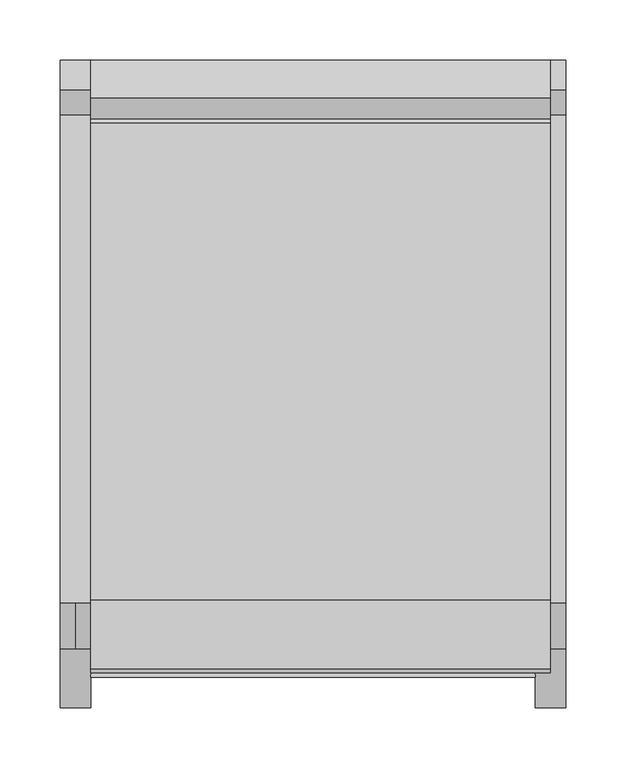
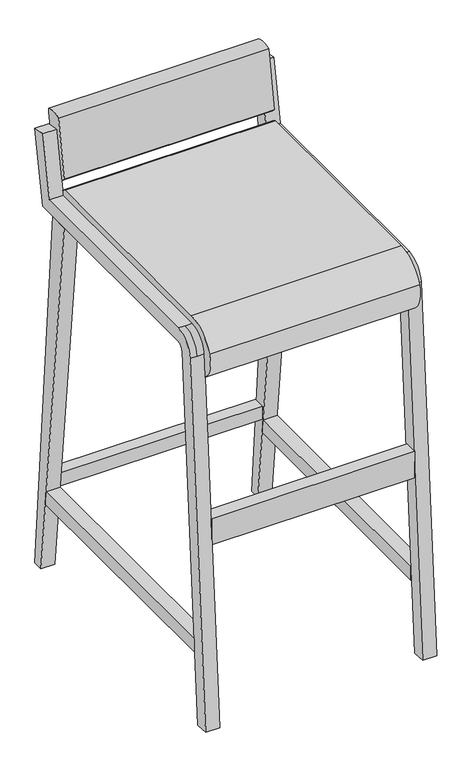
"""IFC4 building model written with IfcOpenShell, lengths in millimetres: furniture geometry, Bar_Stool_6722[1] : Bar_Stool_6722[1]."""

import ifcopenshell
import ifcopenshell.guid

model = None  # the IFC model being written
_history = None  # IfcOwnerHistory: only IFC2X3 demands one
_inside = {}  # id of a spatial element -> (the spatial element, [elements in it])
_under = {}  # id of a project, library or spatial element -> (it, [spatial elements below it])
_declared = {}  # id of a project -> (the project, [libraries it declares])
_typed = {}  # id of a type object -> (the type object, [elements of that type])
_made_of = {}  # id of a material, layer set ... -> (it, [elements and type objects made of it])


def new_model(schema):
    """Start an empty IFC model of exactly this schema.

    Asked for "IFC4X3", IfcOpenShell would pick the latest addendum, in which some entities
    have other attributes; the version numbers below select the first issue.
    IFC2X3 requires an IfcOwnerHistory on every rooted entity: one is made here for all.
    """
    global model, _history
    if schema == "IFC4X3":
        model = ifcopenshell.file(schema_version=(4, 3, 0, 0))
    else:
        model = ifcopenshell.file(schema=schema)
    _inside.clear()
    _under.clear()
    _declared.clear()
    _typed.clear()
    _made_of.clear()
    _history = None
    if model.schema == "IFC2X3":
        org = make("IfcOrganization", Name="unknown")
        user = make(
            "IfcPersonAndOrganization",
            ThePerson=make("IfcPerson", FamilyName="unknown"),
            TheOrganization=org,
        )
        app = make(
            "IfcApplication",
            ApplicationDeveloper=org,
            Version="unknown",
            ApplicationFullName="unknown",
            ApplicationIdentifier="unknown",
        )
        _history = make(
            "IfcOwnerHistory",
            OwningUser=user,
            OwningApplication=app,
            ChangeAction="ADDED",
            CreationDate=0,
        )
    return model


def make(cls, **values):
    """One entity of the class cls with the attributes given. An attribute that is None is left unset."""
    return model.create_entity(
        cls, **{name: value for name, value in values.items() if value is not None}
    )


def rooted(cls, **values):
    """An entity with a GlobalId (a new one), such as an element, a storey or a relation."""
    return make(cls, GlobalId=ifcopenshell.guid.new(), OwnerHistory=_history, **values)


def si_unit(unit_type, name, prefix=None):
    """IfcSIUnit, for example si_unit("LENGTHUNIT", "METRE", prefix="MILLI")."""
    return make("IfcSIUnit", UnitType=unit_type, Prefix=prefix, Name=name)


def assignment(units):
    """IfcUnitAssignment: the units of a project."""
    return None if units is None else make("IfcUnitAssignment", Units=units)


def point(xyz):
    """IfcCartesianPoint."""
    return None if xyz is None else make("IfcCartesianPoint", Coordinates=xyz)


def direction(xyz):
    """IfcDirection."""
    return None if xyz is None else make("IfcDirection", DirectionRatios=xyz)


def frame(location, z_axis=None, x_axis=None):
    """IfcAxis2Placement3D, a coordinate frame: its origin and axes. An axis left out is left unset."""
    return make(
        "IfcAxis2Placement3D",
        Location=point(location),
        Axis=direction(z_axis),
        RefDirection=direction(x_axis),
    )


def frame_2d(location, x_axis=None):
    """IfcAxis2Placement2D, a coordinate frame in the plane: its origin and x axis."""
    return make(
        "IfcAxis2Placement2D", Location=point(location), RefDirection=direction(x_axis)
    )


def origin():
    """The frame at (0, 0, 0) with its axes left unset."""
    return frame((0.0, 0.0, 0.0))


def place(relative_to, where):
    """IfcLocalPlacement: puts the frame where relative to a parent placement (None: the world)."""
    return make(
        "IfcLocalPlacement", PlacementRelTo=relative_to, RelativePlacement=where
    )


def context(
    kind, dimensions, precision=None, world=None, true_north=None, identifier=None
):
    """IfcGeometricRepresentationContext, for example the 3D "Model" context."""
    return make(
        "IfcGeometricRepresentationContext",
        ContextIdentifier=identifier,
        ContextType=kind,
        CoordinateSpaceDimension=dimensions,
        Precision=precision,
        WorldCoordinateSystem=world,
        TrueNorth=true_north,
    )


def project(units=None, contexts=None):
    """IfcProject with its units and contexts."""
    return rooted(
        "IfcProject",
        Name="project",
        RepresentationContexts=contexts,
        UnitsInContext=assignment(units),
    )


def spatial(cls, under=None, at=None, **own):
    """A site, building, storey or space (cls), placed at a placement, below another one or the project."""
    s = rooted(cls, ObjectPlacement=at, **own)
    if under is not None:
        _under.setdefault(under.id(), (under, []))[1].append(s)
    return s


def polyline(points):
    """IfcPolyline through the points."""
    return make("IfcPolyline", Points=[point(p) for p in points])


def circle_curve(where, radius):
    """IfcCircle in the frame where."""
    return make("IfcCircle", Position=where, Radius=radius)


def trimmed(basis, trim1, trim2, sense, master):
    """IfcTrimmedCurve: the piece of a basis curve between two trims."""
    return make(
        "IfcTrimmedCurve",
        BasisCurve=basis,
        Trim1=trim1,
        Trim2=trim2,
        SenseAgreement=sense,
        MasterRepresentation=master,
    )


def segment(curve, same_sense, transition):
    """IfcCompositeCurveSegment."""
    return make(
        "IfcCompositeCurveSegment",
        Transition=transition,
        SameSense=same_sense,
        ParentCurve=curve,
    )


def composite_curve(segments, self_intersect=None):
    """IfcCompositeCurve: segments joined end to end."""
    return make("IfcCompositeCurve", Segments=segments, SelfIntersect=self_intersect)


def outline(outer, holes=None, kind="AREA"):
    """IfcArbitraryClosedProfileDef: a profile drawn as a closed curve; with holes, ...WithVoids."""
    if holes is None:
        return make("IfcArbitraryClosedProfileDef", ProfileType=kind, OuterCurve=outer)
    return make(
        "IfcArbitraryProfileDefWithVoids",
        ProfileType=kind,
        OuterCurve=outer,
        InnerCurves=holes,
    )


def extrude(swept, where, along, depth):
    """IfcExtrudedAreaSolid: the profile swept, set in the frame where, extruded along a direction by depth."""
    return make(
        "IfcExtrudedAreaSolid",
        SweptArea=swept,
        Position=where,
        ExtrudedDirection=direction(along),
        Depth=depth,
    )


def shape(context_of_items, identifier, shape_type, items):
    """IfcShapeRepresentation: the items that make up one representation, for example the "Body"."""
    return make(
        "IfcShapeRepresentation",
        ContextOfItems=context_of_items,
        RepresentationIdentifier=identifier,
        RepresentationType=shape_type,
        Items=items,
    )


def source(mapping_origin, context_of_items, identifier, shape_type, items):
    """IfcRepresentationMap: a shape defined once, which mapped items show again and again."""
    return make(
        "IfcRepresentationMap",
        MappingOrigin=mapping_origin,
        MappedRepresentation=shape(context_of_items, identifier, shape_type, items),
    )


def transform(
    local_origin,
    x_axis=None,
    y_axis=None,
    z_axis=None,
    scale=None,
    scale2=None,
    scale3=None,
    uniform=True,
):
    """IfcCartesianTransformationOperator3D, or its non-uniform kind. x_axis, y_axis, z_axis: its Axis1, 2, 3."""
    if uniform:
        return make(
            "IfcCartesianTransformationOperator3D",
            Axis1=direction(x_axis),
            Axis2=direction(y_axis),
            LocalOrigin=point(local_origin),
            Scale=scale,
            Axis3=direction(z_axis),
        )
    return make(
        "IfcCartesianTransformationOperator3DnonUniform",
        Axis1=direction(x_axis),
        Axis2=direction(y_axis),
        LocalOrigin=point(local_origin),
        Scale=scale,
        Axis3=direction(z_axis),
        Scale2=scale2,
        Scale3=scale3,
    )


def mapped(mapping_source, mapping_target):
    """IfcMappedItem: shows the shape of a source again, moved by a transform."""
    return make(
        "IfcMappedItem", MappingSource=mapping_source, MappingTarget=mapping_target
    )


def made_of(thing, what):
    """Note that an element or type object is made of a material, layer set ...; save() writes the relation."""
    if what is not None:
        _made_of.setdefault(what.id(), (what, []))[1].append(thing)
    return thing


def element(
    cls,
    number,
    at=None,
    inside=None,
    cuts=None,
    type_object=None,
    material=None,
    context=None,
    identifier="Body",
    shape_type=None,
    held_by="IfcProductDefinitionShape",
    body=None,
    shapes=None,
    **own,
):
    """One element of the class cls, such as IfcWall. Its Tag is "e" and its number.

    at: its placement. inside: the storey or other place that contains it. cuts: it is an
    opening in that element (IfcRelVoidsElement). A single representation is given by context,
    identifier, shape_type and body (its items); several are given by shapes. held_by: the class
    of the entity that holds the representations. save() writes the other relations.
    """
    e = rooted(cls, Tag="e%d" % number, ObjectPlacement=at, **own)
    if body is not None:
        shapes = [shape(context, identifier, shape_type, body)]
    if shapes is not None:
        e.Representation = make(held_by, Representations=shapes)
    if inside is not None:
        _inside.setdefault(inside.id(), (inside, []))[1].append(e)
    if cuts is not None:
        rooted(
            "IfcRelVoidsElement", RelatingBuildingElement=cuts, RelatedOpeningElement=e
        )
    if type_object is not None:
        _typed.setdefault(type_object.id(), (type_object, []))[1].append(e)
    return made_of(e, material)


def aggregate(whole, parts):
    """IfcRelAggregates: a whole, such as a stair, and the parts it consists of."""
    return rooted("IfcRelAggregates", RelatingObject=whole, RelatedObjects=parts)


def save(model, path):
    """Write the relations noted so far, then the file.

    IfcRelAggregates (storeys below a building ...), IfcRelContainedInSpatialStructure (elements
    in a storey), IfcRelDefinesByType, IfcRelAssociatesMaterial and IfcRelDeclares: one each for
    every whole, place, type object, material and project.
    """
    for whole, parts in _under.values():
        aggregate(whole, parts)
    for where, things in _inside.values():
        rooted(
            "IfcRelContainedInSpatialStructure",
            RelatedElements=things,
            RelatingStructure=where,
        )
    for kind, things in _typed.values():
        rooted("IfcRelDefinesByType", RelatedObjects=things, RelatingType=kind)
    for what, things in _made_of.values():
        rooted("IfcRelAssociatesMaterial", RelatedObjects=things, RelatingMaterial=what)
    for by, libraries in _declared.values():
        rooted("IfcRelDeclares", RelatingContext=by, RelatedDefinitions=libraries)
    model.write(path)


def plane_surface(at):
    """IfcPlane: the flat surface through the origin of the frame at, square to its z axis."""
    return make("IfcPlane", Position=at)


def cylinder_surface(at, radius):
    """IfcCylindricalSurface: all points at the distance radius from the z axis of the frame at."""
    return make("IfcCylindricalSurface", Position=at, Radius=radius)


def revolved_surface(curve, axis_point, axis_direction):
    """IfcSurfaceOfRevolution: the curve turned about the line through axis_point along axis_direction."""
    return make(
        "IfcSurfaceOfRevolution",
        SweptCurve=make("IfcArbitraryOpenProfileDef", ProfileType="CURVE", Curve=curve),
        AxisPosition=make("IfcAxis1Placement", Location=point(axis_point), Axis=direction(axis_direction)),
    )


def advanced_brep(points, edges, surfaces, faces):
    """IfcAdvancedBrep: a solid bounded by faces that lie on surfaces and meet in shared edges.

    An edge is (start, end): straight between two places in points (the first is 0);
    or (start, end, curve); or (start, end, curve, False) where it runs against its curve.
    A face is (place in surfaces, loops), or (place, loops, False) where it looks against
    its surface's normal. A loop lists edges by number (the first is 1), with a minus sign
    where the edge is run from its end to its start. The first loop is the outer one.
    """
    corners = [point(p) for p in points]
    vertices = [make("IfcVertexPoint", VertexGeometry=c) for c in corners]
    made = []
    for start, end, *more in edges:
        made.append(
            make(
                "IfcEdgeCurve",
                EdgeStart=vertices[start],
                EdgeEnd=vertices[end],
                EdgeGeometry=more[0] if more else make("IfcPolyline", Points=[corners[start], corners[end]]),
                SameSense=more[1] if len(more) > 1 else True,
            )
        )
    hull = []
    for where, loops, *sense in faces:
        bounds = []
        for j, loop in enumerate(loops):
            ring = [make("IfcOrientedEdge", EdgeElement=made[abs(k) - 1], Orientation=k > 0) for k in loop]
            bounds.append(
                make(
                    "IfcFaceOuterBound" if j == 0 else "IfcFaceBound",
                    Bound=make("IfcEdgeLoop", EdgeList=ring),
                    Orientation=True,
                )
            )
        hull.append(make("IfcAdvancedFace", Bounds=bounds, FaceSurface=surfaces[where], SameSense=sense[0] if sense else True))
    return make("IfcAdvancedBrep", Outer=make("IfcClosedShell", CfsFaces=hull))


def furniture_9d95edac(model_context):
    return source(origin(), model_context, "Body", "SolidModel", [
        advanced_brep(
        [(419.1, -25.0141169, 838.4759165), (419.1, 0.0, 834.0652528), (393.7, 0.0, 834.0652528), (393.7, -25.0141169, 838.4759165), (393.7, -45.2169423, 723.9), (419.1, -45.2169423, 723.9), (393.7, -23.9038117, 698.5), (393.7, -450.0350637, 698.5), (393.7, -462.7032819, 686.6979128), (393.7, -511.439502, -0.8979128), (393.7, -536.7759384, 0.8979128), (393.7, -488.0397183, 688.4937383), (393.7, -450.0350637, 723.9), (419.1, -23.9038117, 698.5), (419.1, -450.0350637, 723.9), (419.1, -488.0397183, 688.4937383), (419.1, -536.7759384, 0.8979128), (419.1, -511.439502, -0.8979128), (419.1, -462.7032819, 686.6979128), (419.1, -450.0350637, 698.5), (406.4, -450.0350637, 723.9), (406.4, -488.0397183, 688.4937383)],
        [
            (0, 1),
            (1, 2),
            (2, 3),
            (3, 0),
            (3, 4),
            (4, 5),
            (5, 0),
            (2, 6),
            (6, 7),
            (7, 8, circle_curve(frame((393.7, -450.0350637, 685.8), z_axis=(1.0, 0.0, 0.0), x_axis=(0.0, 0.0, 1.0)), 12.7)),
            (8, 9),
            (9, 10),
            (10, 11),
            (11, 12, circle_curve(frame((393.7, -450.0350637, 685.8), z_axis=(-1.0, 0.0, 0.0), x_axis=(0.0, 0.0, 1.0)), 38.1)),
            (12, 4),
            (1, 13),
            (13, 6),
            (5, 14),
            (14, 15, circle_curve(frame((419.1, -450.0350637, 685.8), z_axis=(1.0, 0.0, 0.0), x_axis=(0.0, 0.0, 1.0)), 38.1)),
            (15, 16),
            (16, 17),
            (17, 18),
            (18, 19, circle_curve(frame((419.1, -450.0350637, 685.8), z_axis=(-1.0, 0.0, 0.0), x_axis=(0.0, 0.0, 1.0)), 12.7)),
            (19, 13),
            (12, 20),
            (20, 14),
            (19, 7),
            (21, 15),
            (20, 21, circle_curve(frame((406.4, -450.0350637, 685.8), z_axis=(1.0, 0.0, 0.0), x_axis=(0.0, 0.0, 1.0)), 38.1)),
            (11, 21),
            (18, 8),
            (10, 16),
            (17, 9),
        ],
        [
            plane_surface(frame((406.4, -12.5070585, 836.2705846), z_axis=(0.0, 0.17364817766692853, 0.9848077530122085), x_axis=(1.0, 0.0, 0.0))),
            plane_surface(frame((406.4, -25.0141169, 838.4759165), z_axis=(0.0, -0.9848077530122085, 0.17364817766692814), x_axis=(0.0, -0.17364817766692814, -0.9848077530122085))),
            plane_surface(frame((393.7, -25.0141169, 838.4759165), z_axis=(-1.0, 0.0, 0.0), x_axis=(0.0, -0.17364817766692808, -0.9848077530122085))),
            plane_surface(frame((393.7, 0.0, 834.0652528), z_axis=(0.0, 0.9848077530122085, -0.17364817766692817), x_axis=(0.0, -0.17364817766692817, -0.9848077530122085))),
            plane_surface(frame((419.1, 0.0, 834.0652528), z_axis=(1.0000000000000002, 0.0, 0.0), x_axis=(0.0, -0.1736481776669284, -0.9848077530122085))),
            plane_surface(frame((406.4, -45.2169423, 723.9), z_axis=(0.0, 0.0, 1.0), x_axis=(0.0, -1.0, 0.0))),
            plane_surface(frame((393.7, -23.9038117, 698.5), z_axis=(0.0, 0.0, -1.0), x_axis=(0.0, -1.0, 0.0))),
            cylinder_surface(frame((406.4, -450.0350637, 685.8), z_axis=(-1.0, 0.0, 0.0), x_axis=(0.0, 0.0, 1.0)), 38.1),
            revolved_surface(polyline([(393.7, -450.0350637, 698.5), (419.1, -450.0350637, 698.5)]), (406.4, -450.0350637, 685.8), (-1.0, 0.0, 0.0)),
            plane_surface(frame((406.4, -488.0397183, 688.4937383), z_axis=(0.0, -0.9974974969901172, 0.07070179275273744), x_axis=(0.0, -0.07070179275273744, -0.9974974969901172))),
            plane_surface(frame((393.7, -462.7032819, 686.6979128), z_axis=(0.0, 0.9974974969901172, -0.07070179275273743), x_axis=(0.0, -0.07070179275273743, -0.9974974969901172))),
            plane_surface(frame((406.4, -524.1077202, 0.0), z_axis=(0.0, -0.07070179275273399, -0.9974974969901175), x_axis=(1.0, 0.0, 0.0))),
        ],
        [
            (0, [[1, 2, 3, 4]]),
            (1, [[-4, 5, 6, 7]]),
            (2, [[8, 9, 10, 11, 12, 13, 14, 15, -5, -3]]),
            (3, [[16, 17, -8, -2]]),
            (4, [[-7, 18, 19, 20, 21, 22, 23, 24, -16, -1]]),
            (5, [[-15, 25, 26, -18, -6]]),
            (6, [[-24, 27, -9, -17]]),
            (7, [[28, -19, -26, 29]]),
            (7, [[30, -29, -25, -14]]),
            (8, [[31, -10, -27, -23]]),
            (9, [[32, -20, -28, -30, -13]]),
            (10, [[33, -11, -31, -22]]),
            (11, [[-12, -33, -21, -32]]),
        ],
    ),
        extrude(outline(composite_curve([segment(polyline([(-48.4096386, 756.5644068), (-31.5225381, 863.1853632)]), True, "CONTINUOUS"), segment(trimmed(circle_curve(frame_2d((-15.7612691, 828.3540875)), 38.2313401), [point((-31.5225381, 863.1853632))], [point((0.0, 863.1853632))], False, "CARTESIAN"), True, "CONTINUOUS"), segment(polyline([(0.0, 863.1853632), (0.0, 856.8353632), (-19.1416957, 748.2774126), (-44.0710693, 752.2258375), (-48.4096386, 756.5644068)]), True, "CONTINUOUS")], self_intersect=False)), frame((25.4, 0.0, 0.0), z_axis=(1.0, 0.0, 0.0), x_axis=(0.0, 1.0, 0.0)), (0.0, 0.0, 1.0), 381.0),
        extrude(outline(composite_curve([segment(polyline([(-51.6744261, 737.5144068), (-43.9498561, 733.0546243), (-46.417441, 704.85), (-452.817441, 704.85), (-460.5585493, 681.23302), (-460.5585493, 643.13302), (-484.2663236, 640.1699505)]), True, "CONTINUOUS"), segment(trimmed(circle_curve(frame_2d((-460.5585493, 681.23302)), 47.4155486), [point((-484.2663236, 640.1699505))], [point((-505.1145904, 697.4500928))], False, "CARTESIAN"), True, "CONTINUOUS"), segment(trimmed(circle_curve(frame_2d((-447.8968201, 676.6245275)), 60.8898793), [point((-505.1145904, 697.4500928))], [point((-447.8968201, 737.5144068))], False, "CARTESIAN"), True, "CONTINUOUS"), segment(polyline([(-447.8968201, 737.5144068), (-51.6744261, 737.5144068)]), True, "CONTINUOUS")], self_intersect=False)), frame((25.4, 0.0, 0.0), z_axis=(1.0, 0.0, 0.0), x_axis=(0.0, 1.0, 0.0)), (0.0, 0.0, 1.0), 381.0),
        extrude(outline(polyline([(393.7, -11.6871233), (393.7, -33.1441574), (25.4, -33.1441574), (25.4, -11.6871233), (393.7, -11.6871233)])), frame((0.0, 0.0, 157.9619127), z_axis=(0.0, 0.0, 1.0), x_axis=(1.0, 0.0, 0.0)), (0.0, 0.0, 1.0), 25.4),
        extrude(outline(polyline([(393.7, -488.2695397), (393.7, -511.439502), (25.4, -511.439502), (25.4, -488.2695397), (393.7, -488.2695397)])), frame((0.0, 0.0, 335.7619127), z_axis=(0.0, 0.0, 1.0), x_axis=(1.0, 0.0, 0.0)), (0.0, 0.0, 1.0), 50.8),
        extrude(outline(polyline([(-500.1796497, 157.9619127), (-35.652466, 157.9619127), (-32.9828185, 132.5619127), (-500.1796497, 132.5619127), (-500.1796497, 157.9619127)])), frame((393.7, 0.0, 0.0), z_axis=(1.0, 0.0, 0.0), x_axis=(0.0, 1.0, 0.0)), (0.0, 0.0, 1.0), 25.4),
        extrude(outline(polyline([(-500.1796497, 157.9619127), (-35.652466, 157.9619127), (-32.9828185, 132.5619127), (-500.1796497, 132.5619127), (-500.1796497, 157.9619127)])), frame((0.0, 0.0, 0.0), z_axis=(1.0, 0.0, 0.0), x_axis=(0.0, 1.0, 0.0)), (0.0, 0.0, 1.0), 25.4),
        extrude(outline(polyline([(0.0, 0.0), (-19.05, 0.0), (-92.4653083, 698.5), (-55.3031462, 698.5), (0.0, 0.0)])), frame((393.7, 0.0, 0.0), z_axis=(1.0, 0.0, 0.0), x_axis=(0.0, 1.0, 0.0)), (0.0, 0.0, 1.0), 25.4),
        advanced_brep(
        [(25.4, -25.0141169, 838.4759165), (25.4, 0.0, 834.0652528), (0.0, 0.0, 834.0652528), (0.0, -25.0141169, 838.4759165), (0.0, -45.2169423, 723.9), (25.4, -45.2169423, 723.9), (0.0, -23.9038117, 698.5), (0.0, -450.0350637, 698.5), (0.0, -462.7032819, 686.6979128), (0.0, -511.439502, -0.8979128), (0.0, -536.7759384, 0.8979128), (0.0, -488.0397183, 688.4937383), (0.0, -450.0350637, 723.9), (25.4, -23.9038117, 698.5), (25.4, -450.0350637, 723.9), (25.4, -488.0397183, 688.4937383), (25.4, -536.7759384, 0.8979128), (25.4, -511.439502, -0.8979128), (25.4, -462.7032819, 686.6979128), (25.4, -450.0350637, 698.5), (12.7, -450.0350637, 723.9), (12.7, -488.0397183, 688.4937383)],
        [
            (0, 1),
            (1, 2),
            (2, 3),
            (3, 0),
            (3, 4),
            (4, 5),
            (5, 0),
            (2, 6),
            (6, 7),
            (7, 8, circle_curve(frame((0.0, -450.0350637, 685.8), z_axis=(1.0, 0.0, 0.0), x_axis=(0.0, 0.0, 1.0)), 12.7)),
            (8, 9),
            (9, 10),
            (10, 11),
            (11, 12, circle_curve(frame((0.0, -450.0350637, 685.8), z_axis=(-1.0, 0.0, 0.0), x_axis=(0.0, 0.0, 1.0)), 38.1)),
            (12, 4),
            (1, 13),
            (13, 6),
            (5, 14),
            (14, 15, circle_curve(frame((25.4, -450.0350637, 685.8), z_axis=(1.0, 0.0, 0.0), x_axis=(0.0, 0.0, 1.0)), 38.1)),
            (15, 16),
            (16, 17),
            (17, 18),
            (18, 19, circle_curve(frame((25.4, -450.0350637, 685.8), z_axis=(-1.0, 0.0, 0.0), x_axis=(0.0, 0.0, 1.0)), 12.7)),
            (19, 13),
            (12, 20),
            (20, 14),
            (19, 7),
            (21, 15),
            (20, 21, circle_curve(frame((12.7, -450.0350637, 685.8), z_axis=(1.0, 0.0, 0.0), x_axis=(0.0, 0.0, 1.0)), 38.1)),
            (11, 21),
            (18, 8),
            (10, 16),
            (17, 9),
        ],
        [
            plane_surface(frame((12.7, -12.5070585, 836.2705846), z_axis=(0.0, 0.17364817766692853, 0.9848077530122085), x_axis=(1.0, 0.0, 0.0))),
            plane_surface(frame((12.7, -25.0141169, 838.4759165), z_axis=(0.0, -0.9848077530122085, 0.173648177666928), x_axis=(0.0, -0.173648177666928, -0.9848077530122085))),
            plane_surface(frame((0.0, -25.0141169, 838.4759165), z_axis=(-1.0, 0.0, 0.0), x_axis=(0.0, -0.17364817766692875, -0.9848077530122084))),
            plane_surface(frame((0.0, 0.0, 834.0652528), z_axis=(0.0, 0.9848077530122084, -0.17364817766692883), x_axis=(0.0, -0.17364817766692883, -0.9848077530122084))),
            plane_surface(frame((25.4, 0.0, 834.0652528), z_axis=(1.0000000000000002, 0.0, 0.0), x_axis=(0.0, -0.1736481776669284, -0.9848077530122085))),
            plane_surface(frame((12.7, -45.2169423, 723.9), z_axis=(0.0, 0.0, 1.0), x_axis=(0.0, -1.0, 0.0))),
            plane_surface(frame((0.0, -23.9038117, 698.5), z_axis=(0.0, 0.0, -1.0), x_axis=(0.0, -1.0, 0.0))),
            cylinder_surface(frame((12.7, -450.0350637, 685.8), z_axis=(-1.0, 0.0, 0.0), x_axis=(0.0, 0.0, 1.0)), 38.1),
            revolved_surface(polyline([(0.0, -450.0350637, 698.5), (25.4, -450.0350637, 698.5)]), (12.7, -450.0350637, 685.8), (-1.0, 0.0, 0.0)),
            plane_surface(frame((12.7, -488.0397183, 688.4937383), z_axis=(0.0, -0.9974974969901172, 0.07070179275273744), x_axis=(0.0, -0.07070179275273744, -0.9974974969901172))),
            plane_surface(frame((0.0, -462.7032819, 686.6979128), z_axis=(0.0, 0.9974974969901172, -0.07070179275273743), x_axis=(0.0, -0.07070179275273743, -0.9974974969901172))),
            plane_surface(frame((12.7, -524.1077202, 0.0), z_axis=(0.0, -0.07070179275273399, -0.9974974969901175), x_axis=(1.0, 0.0, 0.0))),
        ],
        [
            (0, [[1, 2, 3, 4]]),
            (1, [[-4, 5, 6, 7]]),
            (2, [[8, 9, 10, 11, 12, 13, 14, 15, -5, -3]]),
            (3, [[16, 17, -8, -2]]),
            (4, [[-7, 18, 19, 20, 21, 22, 23, 24, -16, -1]]),
            (5, [[-15, 25, 26, -18, -6]]),
            (6, [[-24, 27, -9, -17]]),
            (7, [[28, -19, -26, 29]]),
            (7, [[30, -29, -25, -14]]),
            (8, [[31, -10, -27, -23]]),
            (9, [[32, -20, -28, -30, -13]]),
            (10, [[33, -11, -31, -22]]),
            (11, [[-12, -33, -21, -32]]),
        ],
    ),
        extrude(outline(polyline([(0.0, 0.0), (-19.05, 0.0), (-92.4653083, 698.5), (-55.3031462, 698.5), (0.0, 0.0)])), frame((0.0, 0.0, 0.0), z_axis=(1.0, 0.0, 0.0), x_axis=(0.0, 1.0, 0.0)), (0.0, 0.0, 1.0), 25.4),
    ])


if __name__ == "__main__":
    model = new_model("IFC4")
    model_context = context("Model", 3, world=origin())
    ifc_project = project(units=[si_unit("LENGTHUNIT", "METRE", prefix="MILLI")], contexts=[model_context])
    site = spatial("IfcSite", under=ifc_project)
    building = spatial("IfcBuilding", under=site)
    placement = place(None, origin())
    furniture_shape = furniture_9d95edac(model_context)
    element("IfcFurniture", 1, ObjectType="Bar_Stool_6722[1] : Bar_Stool_6722[1]", at=placement, inside=building, context=model_context, shape_type="MappedRepresentation", body=[
        mapped(furniture_shape, transform((0.0, 0.0, 0.0), x_axis=(1.0, 0.0, 0.0), y_axis=(0.0, 1.0, 0.0), z_axis=(0.0, 0.0, 1.0))),
    ])
    save(model, "model.ifc")

# Revit data of these elements
# Type "Bar_Stool_6722[1] : Bar_Stool_6722[1]"
#   Seat = fab
#   Chair Legs = MET
# Element 1 (IfcFurniture, "Bar_Stool_6722[1] : Bar_Stool_6722[1]")
#   Materials on its faces: "MET", "fab"
# Materials
#   "fab": class "Leather", colour RGB 255 255 255, transparency 0, Cost = 0
#   "MET": class "Metal", colour RGB 189 187 185, transparency 0
